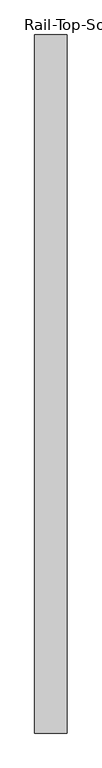
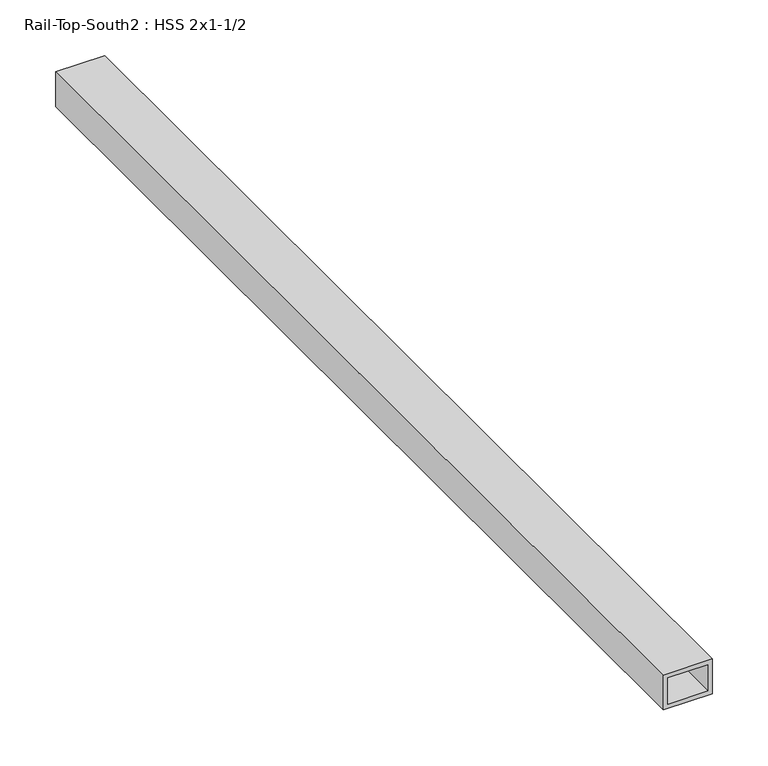
"""IFC4 building model written with IfcOpenShell, lengths in millimetres: proxy geometry, Rail-Top-South2 : HSS 2x1-1/2."""

from ifc_helpers import new_model, si_unit, frame, origin, place, context, project, spatial, polyline, outline, extrude, source, transform, mapped, element, save


def rail_top_south2_hss_2x1_1_2_0885d97b(model_context):
    return source(origin(), model_context, "Body", "SweptSolid", [
        extrude(outline(polyline([(2400.3, 587416.6934739), (2438.4, 587416.6934739), (2438.4, 587365.8934739), (2400.3, 587365.8934739), (2400.3, 587416.6934739)]), holes=[polyline([(2433.6375, 587411.9309739), (2405.0625, 587411.9309739), (2405.0625, 587370.6559739), (2433.6375, 587370.6559739), (2433.6375, 587411.9309739)])]), frame((0.0, -533976.0163841, 0.0), z_axis=(0.0, 1.0, 0.0), x_axis=(0.0, 0.0, 1.0)), (0.0, 0.0, 1.0), 1092.2),
    ])


if __name__ == "__main__":
    model = new_model("IFC4")
    model_context = context("Model", 3, world=origin())
    ifc_project = project(units=[si_unit("LENGTHUNIT", "METRE", prefix="MILLI")], contexts=[model_context])
    site = spatial("IfcSite", under=ifc_project)
    building = spatial("IfcBuilding", under=site)
    placement = place(None, origin())
    rail_top_south2_hss_2x1_1_2_shape = rail_top_south2_hss_2x1_1_2_0885d97b(model_context)
    element("IfcBuildingElementProxy", 1, Name="Rail-Top-South2 : HSS 2x1-1/2", ObjectType="Rail-Top-South2 : HSS 2x1-1/2", at=placement, inside=building, context=model_context, shape_type="MappedRepresentation", body=[
        mapped(rail_top_south2_hss_2x1_1_2_shape, transform((0.0, 0.0, 0.0), x_axis=(1.0, 0.0, 0.0), y_axis=(0.0, 1.0, 0.0), z_axis=(0.0, 0.0, 1.0))),
    ])
    save(model, "model.ifc")

# Revit data of these elements
# Element 1 (IfcBuildingElementProxy, "Rail-Top-South2 : HSS 2x1-1/2")
#   Materials on its faces: "1-1/2\"X2\" GALV. STL HSS TUBING"
# Materials
#   "1-1/2\"X2\" GALV. STL HSS TUBING": class "Generic", colour RGB 211 211 207, transparency 0, Cost = 0
